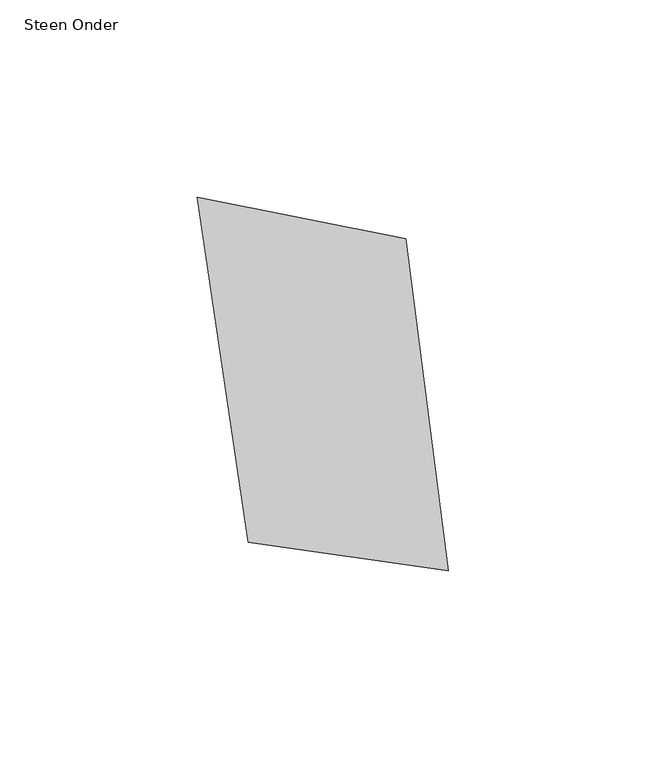
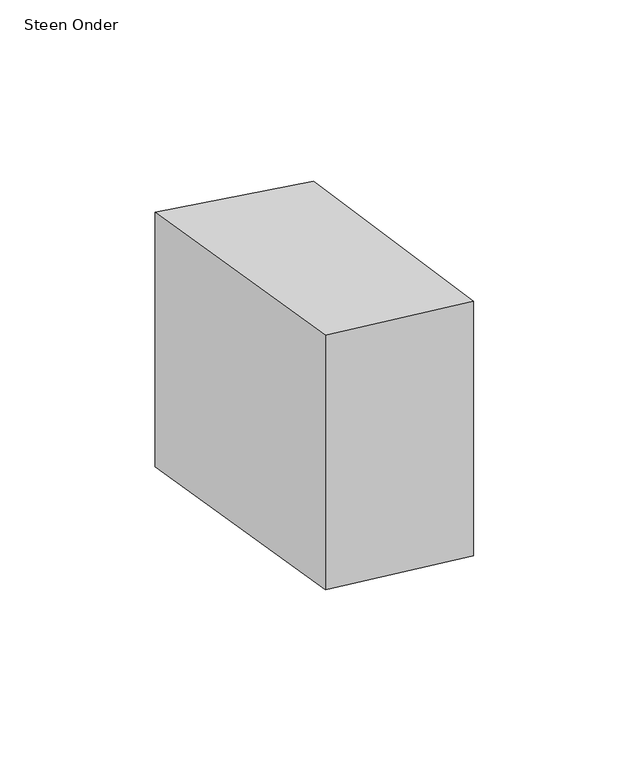
"""IFC4 building model written with IfcOpenShell, lengths in millimetres: proxy geometry, 00_GMA_steen_versie_4 : Steen Onder."""

from ifc_helpers import new_model, si_unit, origin, origin_with_axes, place, context, project, spatial, polyline, outline, extrude, source, transform, mapped, element, save


def steen_onder_e21fbc75(model_context):
    return source(origin(), model_context, "Body", "SweptSolid", [
        extrude(outline(polyline([(95.5270567, 109.0966998), (106.3859335, 24.9276619), (55.6125228, 32.2144469), (42.6526844, 119.6647136), (95.5270567, 109.0966998)])), origin_with_axes(), (0.0, 0.0, 1.0), 100.0),
    ])


if __name__ == "__main__":
    model = new_model("IFC4")
    model_context = context("Model", 3, world=origin())
    ifc_project = project(units=[si_unit("LENGTHUNIT", "METRE", prefix="MILLI")], contexts=[model_context])
    site = spatial("IfcSite", under=ifc_project)
    building = spatial("IfcBuilding", under=site)
    placement = place(None, origin())
    steen_onder_shape = steen_onder_e21fbc75(model_context)
    element("IfcBuildingElementProxy", 1, Name="00_GMA_steen_versie_4 : Steen Onder", ObjectType="00_GMA_steen_versie_4 : Steen Onder", at=placement, inside=building, context=model_context, shape_type="MappedRepresentation", body=[
        mapped(steen_onder_shape, transform((0.0, 0.0, 0.0), x_axis=(1.0, 0.0, 0.0), y_axis=(0.0, 1.0, 0.0), z_axis=(0.0, 0.0, 1.0))),
    ])
    save(model, "model.ifc")

# Revit data of these elements
# Type "00_GMA_steen_versie_4 : Steen Onder"
#   StootVoegHalfBoven [instance default] = 5 mm
#   StootVoegHalf [instance default] = 5 mm
#   StootVoegBreedteOnder = 10 mm
#   StootVoegBreedteBoven = 10 mm
#   Steendikte = 100 mm
#   LintVoegOnderHalf = 0 mm
#   LintVoegOnder = 0 mm
#   LintVoegBovenHalf = 5 mm
#   LintVoegBoven = 10 mm
#   materiaal = none
#   MateriaalVoeg = none
#   Default Elevation = 0
